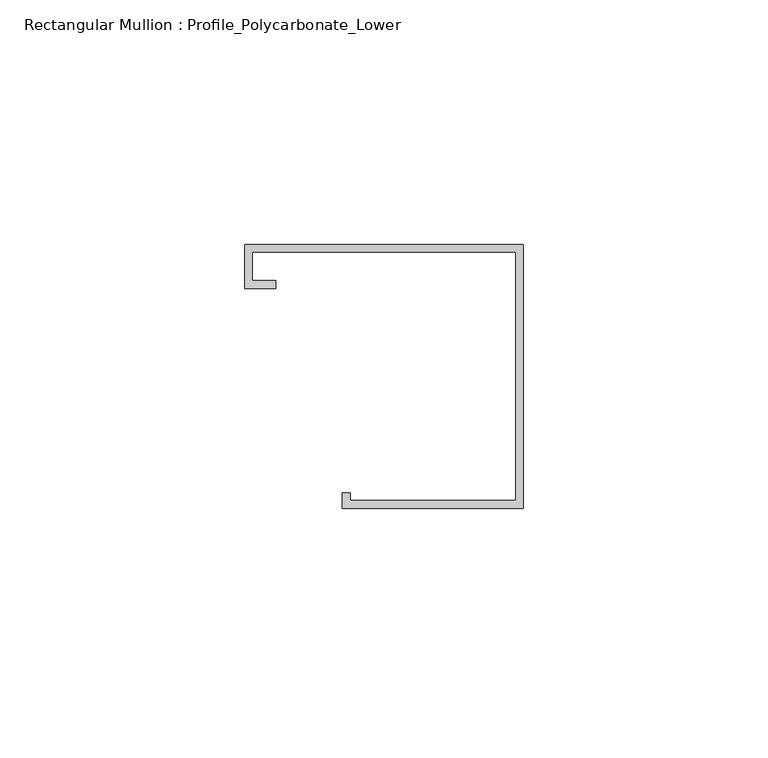
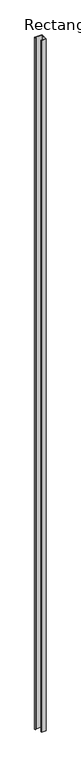
"""IFC4 building model written with IfcOpenShell, lengths in millimetres: member geometry, Rectangular Mullion : Profile_Polycarbonate_Lower."""

from ifc_helpers import new_model, si_unit, frame, origin, place, context, project, spatial, polyline, outline, extrude, source, transform, mapped, element, save


def rectangular_mullion_profile_polycarbonate_lower_5c327cae(model_context):
    return source(origin(), model_context, "Body", "SweptSolid", [
        extrude(outline(polyline([(0.0, 28.984575), (0.0, -25.015825), (-36.9824, -25.015825), (-36.9824, -21.840825), (-35.3949, -21.840825), (-35.3949, -23.428325), (-1.5875, -23.428325), (-1.5875, 27.397075), (-55.4101, 27.397075), (-55.4101, 21.580475), (-50.6476, 21.580475), (-50.6476, 19.992975), (-56.9976, 19.992975), (-56.9976, 28.984575), (0.0, 28.984575)])), frame((0.0, 0.0, -5565.9274), z_axis=(0.0, 0.0, 1.0), x_axis=(1.0, 0.0, 0.0)), (0.0, 0.0, 1.0), 5565.9274),
    ])


if __name__ == "__main__":
    model = new_model("IFC4")
    model_context = context("Model", 3, world=origin())
    ifc_project = project(units=[si_unit("LENGTHUNIT", "METRE", prefix="MILLI")], contexts=[model_context])
    site = spatial("IfcSite", under=ifc_project)
    building = spatial("IfcBuilding", under=site)
    placement = place(None, origin())
    rectangular_mullion_profile_polycarbonate_lower_shape = rectangular_mullion_profile_polycarbonate_lower_5c327cae(model_context)
    element("IfcMember", 1, ObjectType="Rectangular Mullion : Profile_Polycarbonate_Lower", at=placement, inside=building, context=model_context, shape_type="MappedRepresentation", body=[
        mapped(rectangular_mullion_profile_polycarbonate_lower_shape, transform((0.0, 0.0, 0.0), x_axis=(1.0, 0.0, 0.0), y_axis=(0.0, 1.0, 0.0), z_axis=(0.0, 0.0, 1.0))),
    ])
    save(model, "model.ifc")

# Revit data of these elements
# Type "Rectangular Mullion : Profile_Polycarbonate_Lower"
#   built-in parameter 1007322 = 0.177167 (stored number, unit not read)
#   built-in parameter 1007321 = 0 (stored number, unit not read)
#   built-in parameter 1007320 = 0.00520833 (stored number, unit not read)
